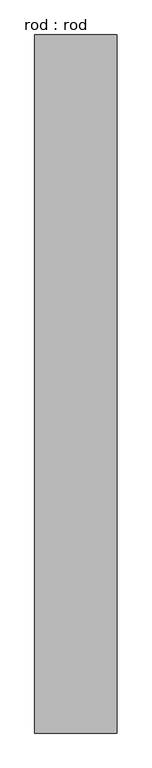
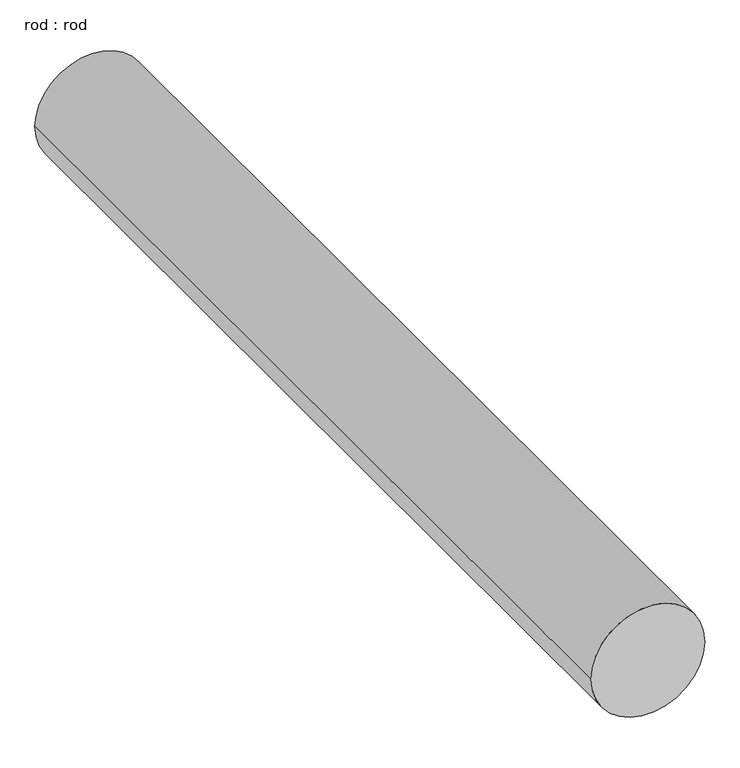
"""IFC4 building model written with IfcOpenShell, lengths in millimetres: proxy geometry, rod : rod."""

from ifc_helpers import new_model, si_unit, point, frame, frame_2d, origin, place, context, project, spatial, circle_curve, trimmed, segment, composite_curve, outline, extrude, source, transform, mapped, element, save


def rod_rod_2dfdf589(model_context):
    return source(origin(), model_context, "Body", "SweptSolid", [
        extrude(outline(composite_curve([segment(trimmed(circle_curve(frame_2d((0.0108462, 0.0)), 200.0), [point((0.0108462, 200.0))], [point((0.0108462, -200.0))], False, "CARTESIAN"), True, "CONTINUOUS"), segment(trimmed(circle_curve(frame_2d((0.0108462, 0.0)), 200.0), [point((0.0108462, -200.0))], [point((0.0108462, 200.0))], False, "CARTESIAN"), True, "CONTINUOUS")], self_intersect=False)), frame((0.0, 2399.8714725, 0.0), z_axis=(0.0, 1.0, 0.0), x_axis=(0.0, 0.0, 1.0)), (0.0, 0.0, 1.0), 3385.7142857),
    ])


if __name__ == "__main__":
    model = new_model("IFC4")
    model_context = context("Model", 3, world=origin())
    ifc_project = project(units=[si_unit("LENGTHUNIT", "METRE", prefix="MILLI")], contexts=[model_context])
    site = spatial("IfcSite", under=ifc_project)
    building = spatial("IfcBuilding", under=site)
    placement = place(None, origin())
    rod_rod_shape = rod_rod_2dfdf589(model_context)
    element("IfcBuildingElementProxy", 1, Name="rod : rod", ObjectType="rod : rod", at=placement, inside=building, context=model_context, shape_type="MappedRepresentation", body=[
        mapped(rod_rod_shape, transform((0.0, 0.0, 0.0), x_axis=(1.0, 0.0, 0.0), y_axis=(0.0, 1.0, 0.0), z_axis=(0.0, 0.0, 1.0))),
    ])
    save(model, "model.ifc")

# Revit data of these elements
# Type "rod : rod"
#   Default Elevation = 0
